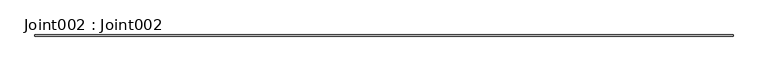
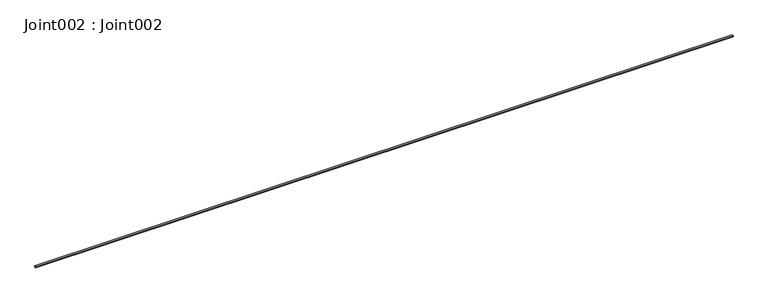
"""IFC4 building model written with IfcOpenShell, lengths in millimetres: proxy geometry, Joint002 : Joint002."""

from ifc_helpers import new_model, si_unit, point, frame, frame_2d, origin, place, context, project, spatial, polyline, circle_curve, trimmed, segment, composite_curve, outline, extrude, source, transform, mapped, element, save


def joint002_joint002_1a41533e(model_context):
    return source(origin(), model_context, "Body", "SweptSolid", [
        extrude(outline(composite_curve([segment(polyline([(9718.4918386, 37509.421875), (9718.4918386, 37513.3398437)]), True, "CONTINUOUS"), segment(trimmed(circle_curve(frame_2d((9720.0901706, 37518.5117187)), 5.4132205), [point((9718.4918386, 37513.3398437))], [point((9721.6885026, 37513.3398437))], True, "CARTESIAN"), True, "CONTINUOUS"), segment(polyline([(9721.6885026, 37513.3398437), (9721.6885026, 37509.421875)]), True, "CONTINUOUS"), segment(trimmed(circle_curve(frame_2d((9720.0901706, 37514.59375)), 5.4132205), [point((9721.6885026, 37509.421875))], [point((9718.4918386, 37509.421875))], False, "CARTESIAN"), True, "CONTINUOUS")], self_intersect=False)), frame((3694.2883192, 0.0, 0.0), z_axis=(1.0, 0.0, 0.0), x_axis=(0.0, 1.0, 0.0)), (0.0, 0.0, 1.0), 2000.0),
    ])


if __name__ == "__main__":
    model = new_model("IFC4")
    model_context = context("Model", 3, world=origin())
    ifc_project = project(units=[si_unit("LENGTHUNIT", "METRE", prefix="MILLI")], contexts=[model_context])
    site = spatial("IfcSite", under=ifc_project)
    building = spatial("IfcBuilding", under=site)
    placement = place(None, origin())
    joint002_joint002_shape = joint002_joint002_1a41533e(model_context)
    element("IfcBuildingElementProxy", 1, Name="Joint002 : Joint002", ObjectType="Joint002 : Joint002", at=placement, inside=building, context=model_context, shape_type="MappedRepresentation", body=[
        mapped(joint002_joint002_shape, transform((0.0, 0.0, 0.0), x_axis=(1.0, 0.0, 0.0), y_axis=(0.0, 1.0, 0.0), z_axis=(0.0, 0.0, 1.0))),
    ])
    save(model, "model.ifc")

# Revit data of these elements
# Type "Joint002 : Joint002"
#   NameOverride = "Joint002"
# Element 1 (IfcBuildingElementProxy, "Joint002 : Joint002")
#   Materials on its faces: "SEALANT JOINT"
# Materials
#   "SEALANT JOINT": class "Unassigned", colour RGB 142 225 148, transparency 0
